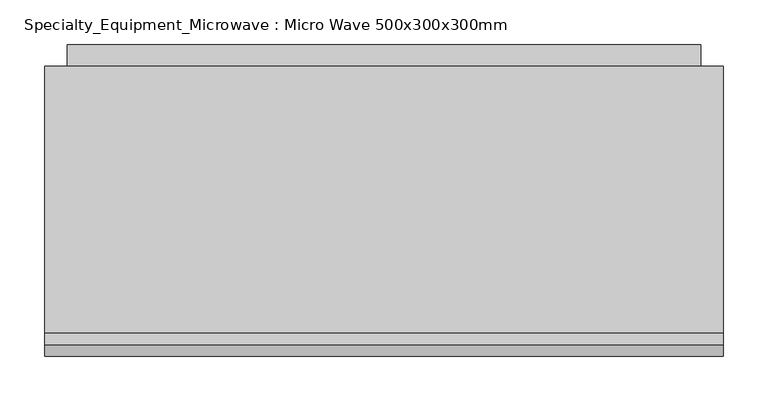
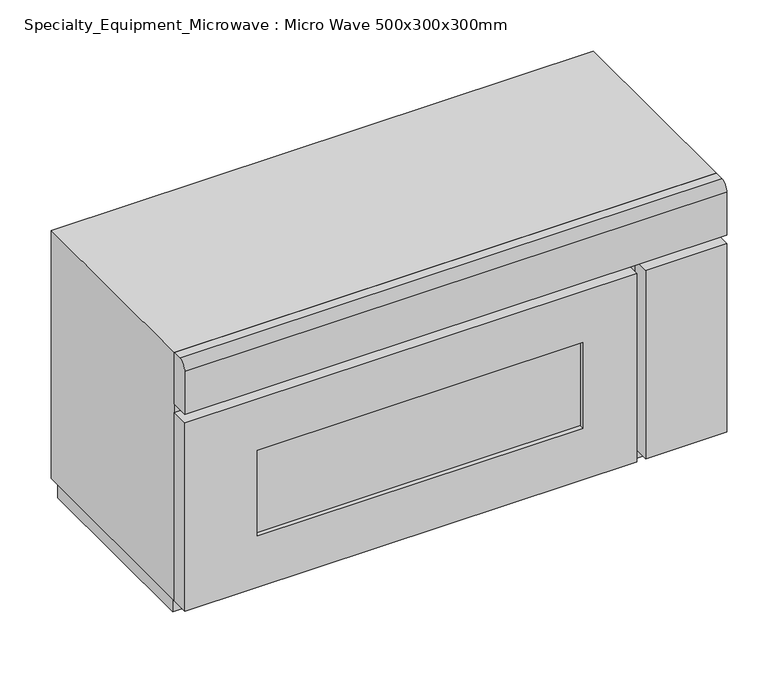
"""IFC4 building model written with IfcOpenShell, lengths in millimetres: proxy geometry, Specialty_Equipment_Microwave : Micro Wave 500x300x300mm."""

from ifc_helpers import new_model, si_unit, point, frame, frame_2d, origin, place, context, project, spatial, polyline, circle_curve, trimmed, segment, composite_curve, outline, extrude, source, transform, mapped, element, save


def specialty_equipment_microwave_micro_wave_500x300x300mm_b58c34cd(model_context):
    return source(origin(), model_context, "Body", "SweptSolid", [
        extrude(outline(polyline([(678.4897523, -521.7305058), (221.8928773, -521.7305058), (221.8928773, -515.3805058), (678.4897523, -515.3805058), (678.4897523, -521.7305058)])), frame((0.0, 0.0, 1022.35), z_axis=(0.0, 0.0, 1.0), x_axis=(1.0, 0.0, 0.0)), (0.0, 0.0, 1.0), 126.95),
        extrude(outline(polyline([(1225.5, 753.6897523), (1225.5, 120.2928773), (946.15, 120.2928773), (946.15, 753.6897523), (1225.5, 753.6897523)]), holes=[polyline([(1149.3, 678.4897523), (1022.35, 678.4897523), (1022.35, 221.8928773), (1149.3, 221.8928773), (1149.3, 678.4897523)])]), frame((0.0, -528.0805058, 0.0), z_axis=(0.0, 1.0, 0.0), x_axis=(0.0, 0.0, 1.0)), (0.0, 0.0, 1.0), 25.4),
        extrude(outline(polyline([(880.2928773, -528.0805058), (766.3897523, -528.0805058), (766.3897523, -502.6805058), (880.2928773, -502.6805058), (880.2928773, -528.0805058)])), frame((0.0, 0.0, 946.15), z_axis=(0.0, 0.0, 1.0), x_axis=(1.0, 0.0, 0.0)), (0.0, 0.0, 1.0), 279.35),
        extrude(outline(composite_curve([segment(polyline([(-515.3805058, 1314.4), (-502.6805058, 1314.4), (-502.6805058, 1238.2), (-528.0805058, 1238.2), (-528.0805058, 1301.7)]), True, "CONTINUOUS"), segment(trimmed(circle_curve(frame_2d((-515.3805058, 1301.7)), 12.7), [point((-528.0805058, 1301.7))], [point((-515.3805058, 1314.4))], False, "CARTESIAN"), True, "CONTINUOUS")], self_intersect=False)), frame((120.2928773, 0.0, 0.0), z_axis=(1.0, 0.0, 0.0), x_axis=(0.0, 1.0, 0.0)), (0.0, 0.0, 1.0), 760.0),
        extrude(outline(polyline([(-179.2441495, 1289.0), (-179.2441495, 961.946551), (-204.6441495, 936.546551), (-204.6441495, 1289.0), (-179.2441495, 1289.0)])), frame((145.6928773, 0.0, 0.0), z_axis=(1.0, 0.0, 0.0), x_axis=(0.0, 1.0, 0.0)), (0.0, 0.0, 1.0), 709.2),
        extrude(outline(polyline([(1314.4, 880.2928773), (1314.4, 120.2928773), (946.15, 120.2928773), (946.15, 880.2928773), (1314.4, 880.2928773)]), holes=[polyline([(1271.0014904, 823.5397523), (1020.1764904, 823.5397523), (1020.1764904, 177.0460023), (1271.0014904, 177.0460023), (1271.0014904, 823.5397523)])]), frame((0.0, -502.6805058, 0.0), z_axis=(0.0, 1.0, 0.0), x_axis=(0.0, 0.0, 1.0)), (0.0, 0.0, 1.0), 299.2),
        extrude(outline(polyline([(870.7678773, -203.4805058), (870.7678773, -482.0430058), (129.8178773, -482.0430058), (129.8178773, -203.4805058), (870.7678773, -203.4805058)])), frame((0.0, 0.0, 914.4), z_axis=(0.0, 0.0, 1.0), x_axis=(1.0, 0.0, 0.0)), (0.0, 0.0, 1.0), 31.75),
    ])


if __name__ == "__main__":
    model = new_model("IFC4")
    model_context = context("Model", 3, world=origin())
    ifc_project = project(units=[si_unit("LENGTHUNIT", "METRE", prefix="MILLI")], contexts=[model_context])
    site = spatial("IfcSite", under=ifc_project)
    building = spatial("IfcBuilding", under=site)
    placement = place(None, origin())
    specialty_equipment_microwave_micro_wave_500x300x300mm_shape = specialty_equipment_microwave_micro_wave_500x300x300mm_b58c34cd(model_context)
    element("IfcBuildingElementProxy", 1, Name="Specialty_Equipment_Microwave : Micro Wave 500x300x300mm", ObjectType="Specialty_Equipment_Microwave : Micro Wave 500x300x300mm", at=placement, inside=building, context=model_context, shape_type="MappedRepresentation", body=[
        mapped(specialty_equipment_microwave_micro_wave_500x300x300mm_shape, transform((0.0, 0.0, 0.0), x_axis=(1.0, 0.0, 0.0), y_axis=(0.0, 1.0, 0.0), z_axis=(0.0, 0.0, 1.0))),
    ])
    save(model, "model.ifc")

# Revit data of these elements
# Type "Specialty_Equipment_Microwave : Micro Wave 500x300x300mm"
#   Keynote = "N"
#   Depth = 350 mm
#   Height = 400 mm
#   Width = 760 mm
#   Material = Laminate - Ivory, Matte
# Element 1 (IfcBuildingElementProxy, "Specialty_Equipment_Microwave : Micro Wave 500x300x300mm")
#   Materials on its faces: "Laminate - Ivory, Matte", "Glass"
# Materials
#   "Laminate - Ivory, Matte": class "Miscellaneous", colour RGB 247 247 239, transparency 0
#   "Glass": class "Glass", colour RGB 0 128 192, transparency 0.9, Description = "Soda Lime Glass", Cost = 0
